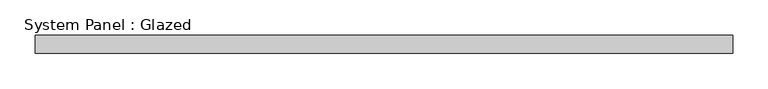
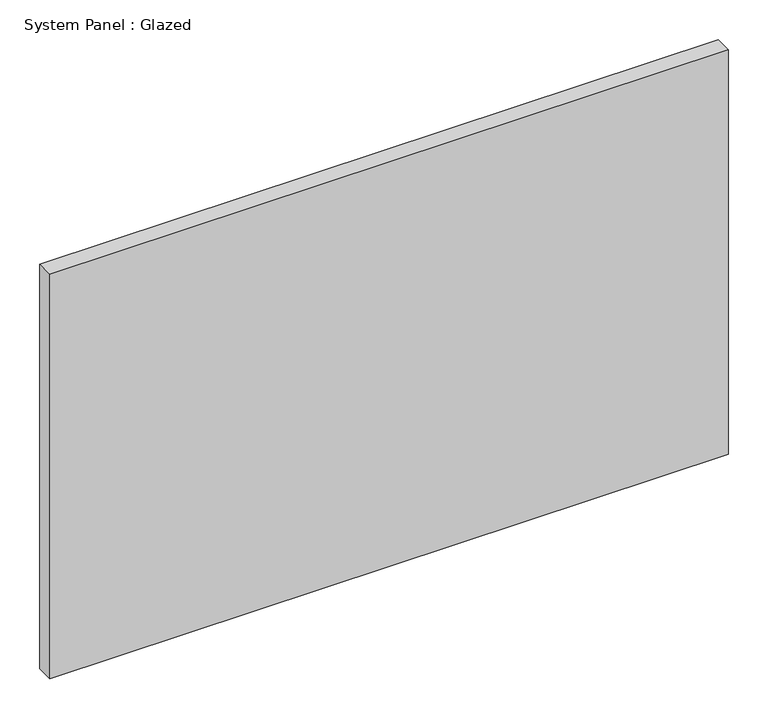
"""IFC4 building model written with IfcOpenShell, lengths in millimetres: plate geometry, System Panel : Glazed."""

from ifc_helpers import new_model, si_unit, origin, origin_with_axes, place, context, project, spatial, polyline, outline, extrude, source, transform, mapped, element, save


def system_panel_glazed_11af89c9(model_context):
    return source(origin(), model_context, "Body", "SweptSolid", [
        extrude(outline(polyline([(493.7595864, 19.05), (-493.7595864, 19.05), (-493.7595864, 44.45), (493.7595864, 44.45), (493.7595864, 19.05)])), origin_with_axes(), (0.0, 0.0, 1.0), 622.3),
    ])


if __name__ == "__main__":
    model = new_model("IFC4")
    model_context = context("Model", 3, world=origin())
    ifc_project = project(units=[si_unit("LENGTHUNIT", "METRE", prefix="MILLI")], contexts=[model_context])
    site = spatial("IfcSite", under=ifc_project)
    building = spatial("IfcBuilding", under=site)
    placement = place(None, origin())
    system_panel_glazed_shape = system_panel_glazed_11af89c9(model_context)
    element("IfcPlate", 1, ObjectType="System Panel : Glazed", at=placement, inside=building, context=model_context, shape_type="MappedRepresentation", body=[
        mapped(system_panel_glazed_shape, transform((0.0, 0.0, 0.0), x_axis=(1.0, 0.0, 0.0), y_axis=(0.0, 1.0, 0.0), z_axis=(0.0, 0.0, 1.0))),
    ])
    save(model, "model.ifc")

# Revit data of these elements
# Element 1 (IfcPlate, "System Panel : Glazed")
#   Materials on its faces: "Glass"
# Materials
#   "Glass": class "Glass", colour RGB 0 128 192, transparency 0.75
